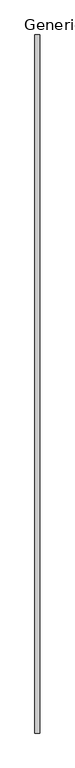
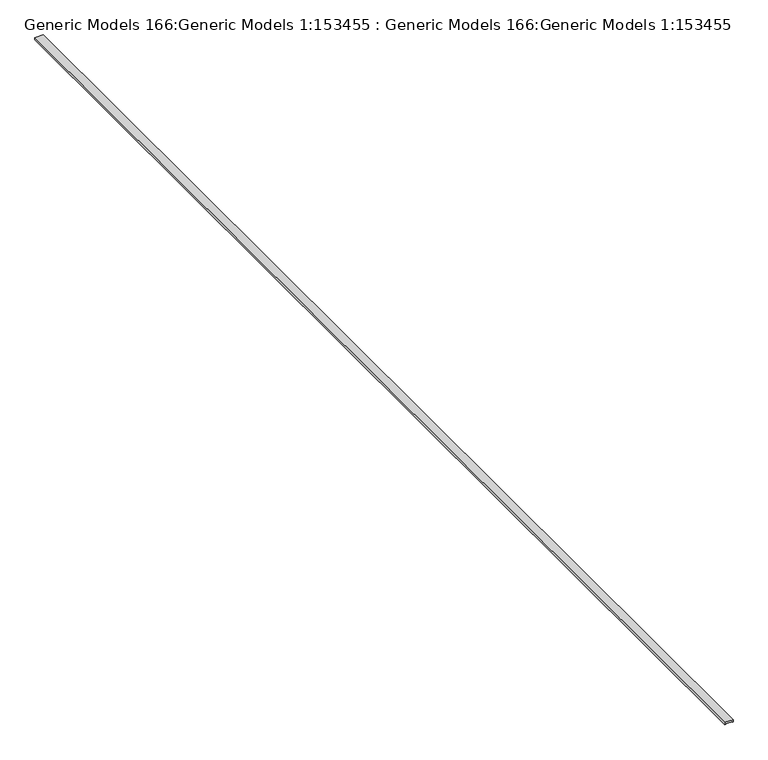
"""IFC4 building model written with IfcOpenShell, lengths in millimetres: proxy geometry, Generic Models 166:Generic Models 1:153455 : Generic Models 166:Generic Models 1:153455."""

from ifc_helpers import new_model, si_unit, frame, origin, place, context, project, spatial, polyline, outline, extrude, source, transform, mapped, element, save


def generic_models_166_generic_models_1_153455_generic_models_55896340(model_context):
    return source(origin(), model_context, "Body", "SweptSolid", [
        extrude(outline(polyline([(830.6782034, -10347.1828813), (849.7282034, -10347.1828813), (849.7282034, -10413.8578813), (830.6782034, -10413.8578813), (830.6782034, -10405.9203813), (837.0282034, -10405.9203813), (837.0282034, -10355.1203813), (830.6782034, -10355.1203813), (830.6782034, -10347.1828813)])), frame((0.0, -464.4974793, 0.0), z_axis=(0.0, 1.0, 0.0), x_axis=(0.0, 0.0, 1.0)), (0.0, 0.0, 1.0), 9475.7774227),
    ])


if __name__ == "__main__":
    model = new_model("IFC4")
    model_context = context("Model", 3, world=origin())
    ifc_project = project(units=[si_unit("LENGTHUNIT", "METRE", prefix="MILLI")], contexts=[model_context])
    site = spatial("IfcSite", under=ifc_project)
    building = spatial("IfcBuilding", under=site)
    placement = place(None, origin())
    generic_models_166_generic_models_1_153455_generic_models_shape = generic_models_166_generic_models_1_153455_generic_models_55896340(model_context)
    element("IfcBuildingElementProxy", 1, Name="Generic Models 166:Generic Models 1:153455 : Generic Models 166:Generic Models 1:153455", ObjectType="Generic Models 166:Generic Models 1:153455 : Generic Models 166:Generic Models 1:153455", at=placement, inside=building, context=model_context, shape_type="MappedRepresentation", body=[
        mapped(generic_models_166_generic_models_1_153455_generic_models_shape, transform((0.0, 0.0, 0.0), x_axis=(1.0, 0.0, 0.0), y_axis=(0.0, 1.0, 0.0), z_axis=(0.0, 0.0, 1.0))),
    ])
    save(model, "model.ifc")

# Revit data of these elements
# Type "Generic Models 166:Generic Models 1:153455 : Generic Models 166:Generic Models 1:153455"
#   NameOverride = "Generic Models 166:Generic Models 1:153455"
#   ObjectTypeOverride = "Generic Models 166:Generic Models 1"
#   Reference = "Generic Models 1"
#   Category = "Generic Models"
#   Tag = "153455"
# Element 1 (IfcBuildingElementProxy, "Generic Models 166:Generic Models 1:153455 : Generic Models 166:Generic Models 1:153455")
#   Materials on its faces: "_2 5/8\" X 3/4\" WOOD TOP RAIL / HAND RAIL, EASE EDGES W/ .01 RADIUS 13878"
# Materials
#   "_2 5/8\" X 3/4\" WOOD TOP RAIL / HAND RAIL, EASE EDGES W/ .01 RADIUS 13878": class "Unassigned", colour RGB 177 130 114, transparency 0
